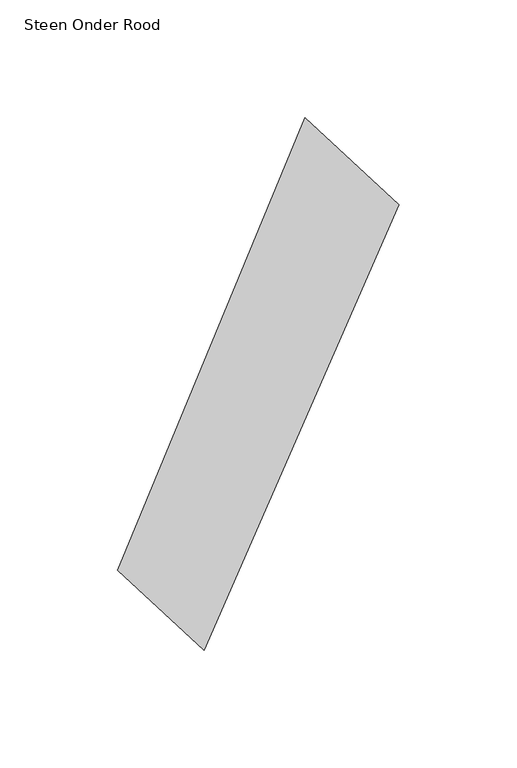
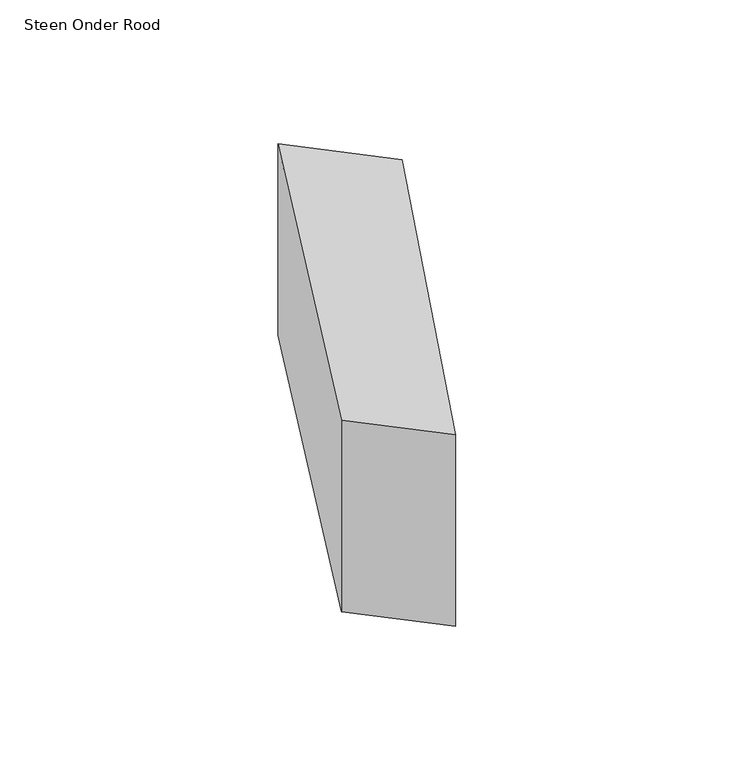
"""IFC4 building model written with IfcOpenShell, lengths in millimetres: proxy geometry, 00_GMA_steen_versie_4 : Steen Onder Rood."""

from ifc_helpers import new_model, si_unit, origin, origin_with_axes, place, context, project, spatial, polyline, outline, extrude, source, transform, mapped, element, save


def steen_onder_rood_b9ab4ce2(model_context):
    return source(origin(), model_context, "Body", "SweptSolid", [
        extrude(outline(polyline([(142.2826817, 164.2955738), (59.4648303, -24.9068775), (22.6870104, 8.9662973), (102.3229888, 201.1372628), (142.2826817, 164.2955738)])), origin_with_axes(), (0.0, 0.0, 1.0), 100.0),
    ])


if __name__ == "__main__":
    model = new_model("IFC4")
    model_context = context("Model", 3, world=origin())
    ifc_project = project(units=[si_unit("LENGTHUNIT", "METRE", prefix="MILLI")], contexts=[model_context])
    site = spatial("IfcSite", under=ifc_project)
    building = spatial("IfcBuilding", under=site)
    placement = place(None, origin())
    steen_onder_rood_shape = steen_onder_rood_b9ab4ce2(model_context)
    element("IfcBuildingElementProxy", 1, Name="00_GMA_steen_versie_4 : Steen Onder Rood", ObjectType="00_GMA_steen_versie_4 : Steen Onder Rood", at=placement, inside=building, context=model_context, shape_type="MappedRepresentation", body=[
        mapped(steen_onder_rood_shape, transform((0.0, 0.0, 0.0), x_axis=(1.0, 0.0, 0.0), y_axis=(0.0, 1.0, 0.0), z_axis=(0.0, 0.0, 1.0))),
    ])
    save(model, "model.ifc")

# Revit data of these elements
# Type "00_GMA_steen_versie_4 : Steen Onder Rood"
#   StootVoegHalfBoven [instance default] = 5 mm
#   StootVoegHalf [instance default] = 5 mm
#   StootVoegBreedteOnder = 10 mm
#   StootVoegBreedteBoven = 10 mm
#   Steendikte = 100 mm
#   LintVoegOnderHalf = 0 mm
#   LintVoegOnder = 0 mm
#   LintVoegBovenHalf = 5 mm
#   LintVoegBoven = 10 mm
#   materiaal = 21_steen_rood
#   MateriaalVoeg = none
#   Default Elevation = 0
# Element 1 (IfcBuildingElementProxy, "00_GMA_steen_versie_4 : Steen Onder Rood")
#   Materials on its faces: "21_steen_rood"
# Materials
#   "21_steen_rood": class "Unassigned", colour RGB 213 111 43, transparency 0, Cost = 0
